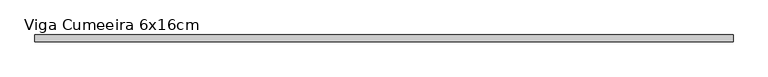
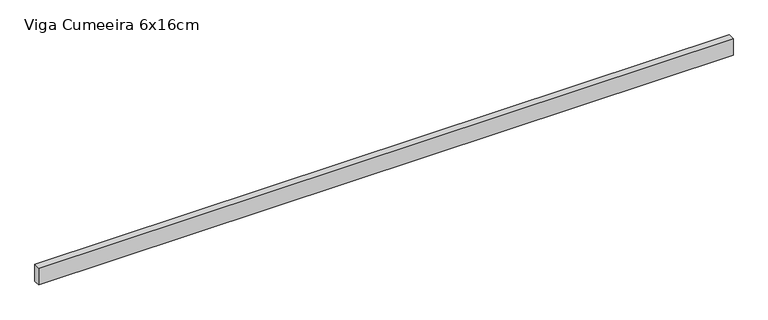
"""IFC4 building model written with IfcOpenShell, lengths in millimetres: beam geometry, Madeira de lei : Viga Cumeeira 6x16cm."""

import ifcopenshell
import ifcopenshell.guid

model = None  # the IFC model being written
_history = None  # IfcOwnerHistory: only IFC2X3 demands one
_inside = {}  # id of a spatial element -> (the spatial element, [elements in it])
_under = {}  # id of a project, library or spatial element -> (it, [spatial elements below it])
_declared = {}  # id of a project -> (the project, [libraries it declares])
_typed = {}  # id of a type object -> (the type object, [elements of that type])
_made_of = {}  # id of a material, layer set ... -> (it, [elements and type objects made of it])


def new_model(schema):
    """Start an empty IFC model of exactly this schema.

    Asked for "IFC4X3", IfcOpenShell would pick the latest addendum, in which some entities
    have other attributes; the version numbers below select the first issue.
    IFC2X3 requires an IfcOwnerHistory on every rooted entity: one is made here for all.
    """
    global model, _history
    if schema == "IFC4X3":
        model = ifcopenshell.file(schema_version=(4, 3, 0, 0))
    else:
        model = ifcopenshell.file(schema=schema)
    _inside.clear()
    _under.clear()
    _declared.clear()
    _typed.clear()
    _made_of.clear()
    _history = None
    if model.schema == "IFC2X3":
        org = make("IfcOrganization", Name="unknown")
        user = make(
            "IfcPersonAndOrganization",
            ThePerson=make("IfcPerson", FamilyName="unknown"),
            TheOrganization=org,
        )
        app = make(
            "IfcApplication",
            ApplicationDeveloper=org,
            Version="unknown",
            ApplicationFullName="unknown",
            ApplicationIdentifier="unknown",
        )
        _history = make(
            "IfcOwnerHistory",
            OwningUser=user,
            OwningApplication=app,
            ChangeAction="ADDED",
            CreationDate=0,
        )
    return model


def make(cls, **values):
    """One entity of the class cls with the attributes given. An attribute that is None is left unset."""
    return model.create_entity(
        cls, **{name: value for name, value in values.items() if value is not None}
    )


def rooted(cls, **values):
    """An entity with a GlobalId (a new one), such as an element, a storey or a relation."""
    return make(cls, GlobalId=ifcopenshell.guid.new(), OwnerHistory=_history, **values)


def si_unit(unit_type, name, prefix=None):
    """IfcSIUnit, for example si_unit("LENGTHUNIT", "METRE", prefix="MILLI")."""
    return make("IfcSIUnit", UnitType=unit_type, Prefix=prefix, Name=name)


def assignment(units):
    """IfcUnitAssignment: the units of a project."""
    return None if units is None else make("IfcUnitAssignment", Units=units)


def point(xyz):
    """IfcCartesianPoint."""
    return None if xyz is None else make("IfcCartesianPoint", Coordinates=xyz)


def direction(xyz):
    """IfcDirection."""
    return None if xyz is None else make("IfcDirection", DirectionRatios=xyz)


def frame(location, z_axis=None, x_axis=None):
    """IfcAxis2Placement3D, a coordinate frame: its origin and axes. An axis left out is left unset."""
    return make(
        "IfcAxis2Placement3D",
        Location=point(location),
        Axis=direction(z_axis),
        RefDirection=direction(x_axis),
    )


def origin():
    """The frame at (0, 0, 0) with its axes left unset."""
    return frame((0.0, 0.0, 0.0))


def place(relative_to, where):
    """IfcLocalPlacement: puts the frame where relative to a parent placement (None: the world)."""
    return make(
        "IfcLocalPlacement", PlacementRelTo=relative_to, RelativePlacement=where
    )


def context(
    kind, dimensions, precision=None, world=None, true_north=None, identifier=None
):
    """IfcGeometricRepresentationContext, for example the 3D "Model" context."""
    return make(
        "IfcGeometricRepresentationContext",
        ContextIdentifier=identifier,
        ContextType=kind,
        CoordinateSpaceDimension=dimensions,
        Precision=precision,
        WorldCoordinateSystem=world,
        TrueNorth=true_north,
    )


def project(units=None, contexts=None):
    """IfcProject with its units and contexts."""
    return rooted(
        "IfcProject",
        Name="project",
        RepresentationContexts=contexts,
        UnitsInContext=assignment(units),
    )


def spatial(cls, under=None, at=None, **own):
    """A site, building, storey or space (cls), placed at a placement, below another one or the project."""
    s = rooted(cls, ObjectPlacement=at, **own)
    if under is not None:
        _under.setdefault(under.id(), (under, []))[1].append(s)
    return s


def polyline(points):
    """IfcPolyline through the points."""
    return make("IfcPolyline", Points=[point(p) for p in points])


def outline(outer, holes=None, kind="AREA"):
    """IfcArbitraryClosedProfileDef: a profile drawn as a closed curve; with holes, ...WithVoids."""
    if holes is None:
        return make("IfcArbitraryClosedProfileDef", ProfileType=kind, OuterCurve=outer)
    return make(
        "IfcArbitraryProfileDefWithVoids",
        ProfileType=kind,
        OuterCurve=outer,
        InnerCurves=holes,
    )


def extrude(swept, where, along, depth):
    """IfcExtrudedAreaSolid: the profile swept, set in the frame where, extruded along a direction by depth."""
    return make(
        "IfcExtrudedAreaSolid",
        SweptArea=swept,
        Position=where,
        ExtrudedDirection=direction(along),
        Depth=depth,
    )


def shape(context_of_items, identifier, shape_type, items):
    """IfcShapeRepresentation: the items that make up one representation, for example the "Body"."""
    return make(
        "IfcShapeRepresentation",
        ContextOfItems=context_of_items,
        RepresentationIdentifier=identifier,
        RepresentationType=shape_type,
        Items=items,
    )


def source(mapping_origin, context_of_items, identifier, shape_type, items):
    """IfcRepresentationMap: a shape defined once, which mapped items show again and again."""
    return make(
        "IfcRepresentationMap",
        MappingOrigin=mapping_origin,
        MappedRepresentation=shape(context_of_items, identifier, shape_type, items),
    )


def transform(
    local_origin,
    x_axis=None,
    y_axis=None,
    z_axis=None,
    scale=None,
    scale2=None,
    scale3=None,
    uniform=True,
):
    """IfcCartesianTransformationOperator3D, or its non-uniform kind. x_axis, y_axis, z_axis: its Axis1, 2, 3."""
    if uniform:
        return make(
            "IfcCartesianTransformationOperator3D",
            Axis1=direction(x_axis),
            Axis2=direction(y_axis),
            LocalOrigin=point(local_origin),
            Scale=scale,
            Axis3=direction(z_axis),
        )
    return make(
        "IfcCartesianTransformationOperator3DnonUniform",
        Axis1=direction(x_axis),
        Axis2=direction(y_axis),
        LocalOrigin=point(local_origin),
        Scale=scale,
        Axis3=direction(z_axis),
        Scale2=scale2,
        Scale3=scale3,
    )


def mapped(mapping_source, mapping_target):
    """IfcMappedItem: shows the shape of a source again, moved by a transform."""
    return make(
        "IfcMappedItem", MappingSource=mapping_source, MappingTarget=mapping_target
    )


def made_of(thing, what):
    """Note that an element or type object is made of a material, layer set ...; save() writes the relation."""
    if what is not None:
        _made_of.setdefault(what.id(), (what, []))[1].append(thing)
    return thing


def element(
    cls,
    number,
    at=None,
    inside=None,
    cuts=None,
    type_object=None,
    material=None,
    context=None,
    identifier="Body",
    shape_type=None,
    held_by="IfcProductDefinitionShape",
    body=None,
    shapes=None,
    **own,
):
    """One element of the class cls, such as IfcWall. Its Tag is "e" and its number.

    at: its placement. inside: the storey or other place that contains it. cuts: it is an
    opening in that element (IfcRelVoidsElement). A single representation is given by context,
    identifier, shape_type and body (its items); several are given by shapes. held_by: the class
    of the entity that holds the representations. save() writes the other relations.
    """
    e = rooted(cls, Tag="e%d" % number, ObjectPlacement=at, **own)
    if body is not None:
        shapes = [shape(context, identifier, shape_type, body)]
    if shapes is not None:
        e.Representation = make(held_by, Representations=shapes)
    if inside is not None:
        _inside.setdefault(inside.id(), (inside, []))[1].append(e)
    if cuts is not None:
        rooted(
            "IfcRelVoidsElement", RelatingBuildingElement=cuts, RelatedOpeningElement=e
        )
    if type_object is not None:
        _typed.setdefault(type_object.id(), (type_object, []))[1].append(e)
    return made_of(e, material)


def aggregate(whole, parts):
    """IfcRelAggregates: a whole, such as a stair, and the parts it consists of."""
    return rooted("IfcRelAggregates", RelatingObject=whole, RelatedObjects=parts)


def save(model, path):
    """Write the relations noted so far, then the file.

    IfcRelAggregates (storeys below a building ...), IfcRelContainedInSpatialStructure (elements
    in a storey), IfcRelDefinesByType, IfcRelAssociatesMaterial and IfcRelDeclares: one each for
    every whole, place, type object, material and project.
    """
    for whole, parts in _under.values():
        aggregate(whole, parts)
    for where, things in _inside.values():
        rooted(
            "IfcRelContainedInSpatialStructure",
            RelatedElements=things,
            RelatingStructure=where,
        )
    for kind, things in _typed.values():
        rooted("IfcRelDefinesByType", RelatedObjects=things, RelatingType=kind)
    for what, things in _made_of.values():
        rooted("IfcRelAssociatesMaterial", RelatedObjects=things, RelatingMaterial=what)
    for by, libraries in _declared.values():
        rooted("IfcRelDeclares", RelatingContext=by, RelatedDefinitions=libraries)
    model.write(path)


def viga_cumeeira_6x16cm_e360fa9d(model_context):
    return source(origin(), model_context, "Body", "SweptSolid", [
        extrude(outline(polyline([(3133.5, 30.0), (3133.5, -30.0), (-3133.5, -30.0), (-3133.5, 30.0), (3133.5, 30.0)])), frame((0.0, 0.0, -80.0), z_axis=(0.0, 0.0, 1.0), x_axis=(1.0, 0.0, 0.0)), (0.0, 0.0, 1.0), 160.0),
    ])


if __name__ == "__main__":
    model = new_model("IFC4")
    model_context = context("Model", 3, world=origin())
    ifc_project = project(units=[si_unit("LENGTHUNIT", "METRE", prefix="MILLI")], contexts=[model_context])
    site = spatial("IfcSite", under=ifc_project)
    building = spatial("IfcBuilding", under=site)
    placement = place(None, origin())
    viga_cumeeira_6x16cm_shape = viga_cumeeira_6x16cm_e360fa9d(model_context)
    element("IfcBeam", 1, ObjectType="Madeira de lei : Viga Cumeeira 6x16cm", at=placement, inside=building, context=model_context, shape_type="MappedRepresentation", body=[
        mapped(viga_cumeeira_6x16cm_shape, transform((0.0, 0.0, 0.0), x_axis=(1.0, 0.0, 0.0), y_axis=(0.0, 1.0, 0.0), z_axis=(0.0, 0.0, 1.0))),
    ])
    save(model, "model.ifc")

# Revit data of these elements
# Type "Madeira de lei : Viga Cumeeira 6x16cm"
#   A = 0.02 m²
#   Length [instance default] = 1.524 m
#   b = 0.06 m
#   d = 0.16 m
#   Structural Material [instance default] = none
#   Assembly Code = ""
# Element 1 (IfcBeam, "Madeira de lei : Viga Cumeeira 6x16cm")
#   Structural Material = .MADEIRAMENTO
#   Materials on its faces: ".MADEIRAMENTO"
# Materials
#   ".MADEIRAMENTO": class ".CC_MADEIRAS", colour RGB 212 179 113, transparency 0, Cost = 0
